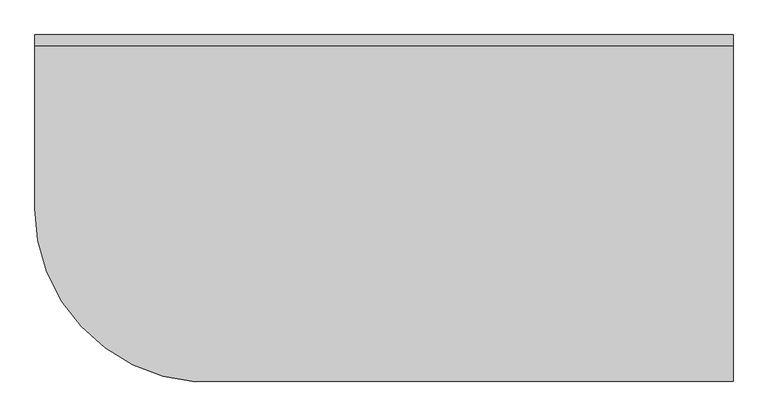
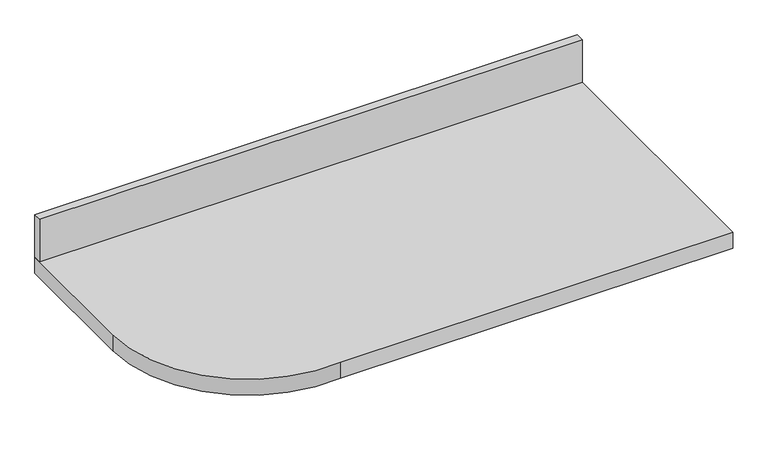
"""IFC4 building model written with IfcOpenShell, lengths in millimetres: furniture geometry, Ketchen counter 1 : Ketchen counter 1."""

from ifc_helpers import new_model, si_unit, point, frame, frame_2d, origin, place, context, project, spatial, polyline, circle_curve, trimmed, segment, composite_curve, outline, extrude, source, transform, mapped, element, save


def furniture_1c508832(model_context):
    return source(origin(), model_context, "Body", "SweptSolid", [
        extrude(outline(polyline([(6102.35, 13469.3107509), (6102.35, 13450.2607509), (4878.0756586, 13450.2607509), (4878.0756586, 13469.3107509), (6102.35, 13469.3107509)])), frame((0.0, 0.0, 914.4), z_axis=(0.0, 0.0, 1.0), x_axis=(1.0, 0.0, 0.0)), (0.0, 0.0, 1.0), 101.6),
        extrude(outline(composite_curve([segment(polyline([(6102.35, 12860.8855304), (5215.6122152, 12860.8855304)]), True, "CONTINUOUS"), segment(trimmed(circle_curve(frame_2d((5183.4043667, 13164.5107509)), 305.3287081), [point((5215.6122152, 12860.8855304))], [point((4878.0756586, 13164.5107509))], False, "CARTESIAN"), True, "CONTINUOUS"), segment(polyline([(4878.0756586, 13164.5107509), (4878.0756586, 13469.3107509), (6102.35, 13469.3107509), (6102.35, 12860.8855304)]), True, "CONTINUOUS")], self_intersect=False)), frame((0.0, 0.0, 876.3), z_axis=(0.0, 0.0, 1.0), x_axis=(1.0, 0.0, 0.0)), (0.0, 0.0, 1.0), 38.1),
    ])


if __name__ == "__main__":
    model = new_model("IFC4")
    model_context = context("Model", 3, world=origin())
    ifc_project = project(units=[si_unit("LENGTHUNIT", "METRE", prefix="MILLI")], contexts=[model_context])
    site = spatial("IfcSite", under=ifc_project)
    building = spatial("IfcBuilding", under=site)
    placement = place(None, origin())
    furniture_shape = furniture_1c508832(model_context)
    element("IfcFurniture", 1, ObjectType="Ketchen counter 1 : Ketchen counter 1", at=placement, inside=building, context=model_context, shape_type="MappedRepresentation", body=[
        mapped(furniture_shape, transform((0.0, 0.0, 0.0), x_axis=(1.0, 0.0, 0.0), y_axis=(0.0, 1.0, 0.0), z_axis=(0.0, 0.0, 1.0))),
    ])
    save(model, "model.ifc")

# Revit data of these elements
# Type "Ketchen counter 1 : Ketchen counter 1"
#   COBie.Type = no
# Element 1 (IfcFurniture, "Ketchen counter 1 : Ketchen counter 1")
#   Materials on its faces: "Corian - Dusk"
# Materials
#   "Corian - Dusk": class "Plastic", colour RGB 75 95 146, transparency 0, Manufacturer = "Corning", Cost = 0
